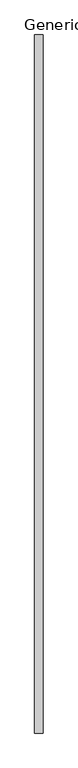
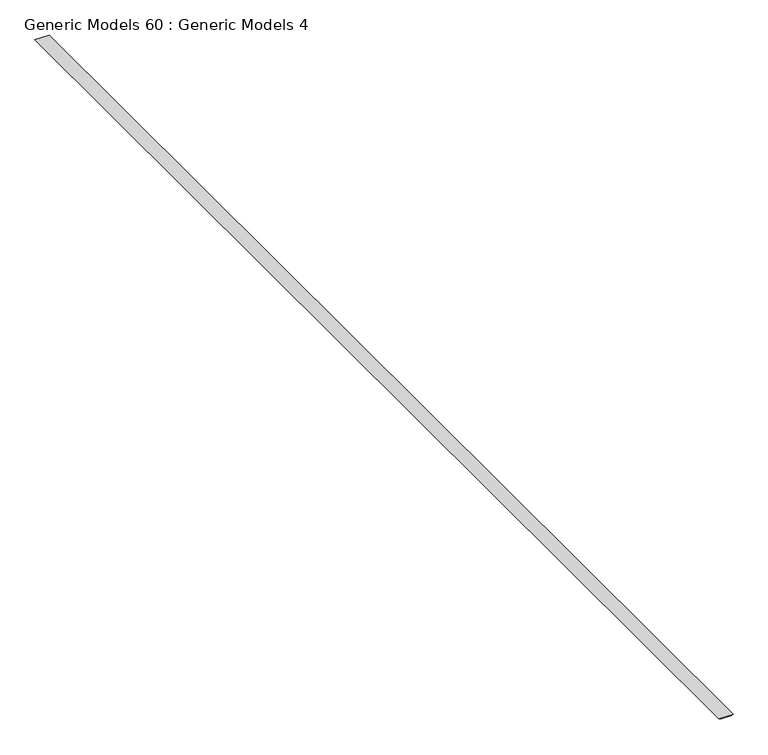
"""IFC4 building model written with IfcOpenShell, lengths in millimetres: proxy geometry, Generic Models 60 : Generic Models 4."""

from ifc_helpers import new_model, si_unit, frame, origin, place, context, project, spatial, polyline, outline, extrude, source, transform, mapped, element, save


def generic_models_60_generic_models_4_e0b604c5(model_context):
    return source(origin(), model_context, "Body", "SweptSolid", [
        extrude(outline(polyline([(126933.5840478, -9268.534981), (126950.6852144, -9235.2327093), (126955.2896197, -9459.8802697), (126936.7665653, -9423.8090585), (126933.5840478, -9268.534981)])), frame((0.0, -6864.9230338, 0.0), z_axis=(0.0, 1.0, 0.0), x_axis=(0.0, 0.0, 1.0)), (0.0, 0.0, 1.0), 18643.6),
    ])


if __name__ == "__main__":
    model = new_model("IFC4")
    model_context = context("Model", 3, world=origin())
    ifc_project = project(units=[si_unit("LENGTHUNIT", "METRE", prefix="MILLI")], contexts=[model_context])
    site = spatial("IfcSite", under=ifc_project)
    building = spatial("IfcBuilding", under=site)
    placement = place(None, origin())
    generic_models_60_generic_models_4_shape = generic_models_60_generic_models_4_e0b604c5(model_context)
    element("IfcBuildingElementProxy", 1, Name="Generic Models 60 : Generic Models 4", ObjectType="Generic Models 60 : Generic Models 4", at=placement, inside=building, context=model_context, shape_type="MappedRepresentation", body=[
        mapped(generic_models_60_generic_models_4_shape, transform((0.0, 0.0, 0.0), x_axis=(1.0, 0.0, 0.0), y_axis=(0.0, 1.0, 0.0), z_axis=(0.0, 0.0, 1.0))),
    ])
    save(model, "model.ifc")

# Revit data of these elements
# Element 1 (IfcBuildingElementProxy, "Generic Models 60 : Generic Models 4")
#   Materials on its faces: "_7/8\" SMOOTH TROWEL EXTERIOR STUCCO (COLOR PER OWNER) @ 2% SLOPE"
# Materials
#   "_7/8\" SMOOTH TROWEL EXTERIOR STUCCO (COLOR PER OWNER) @ 2% SLOPE": class "Generic", colour RGB 233 233 233, transparency 0, Cost = 0
